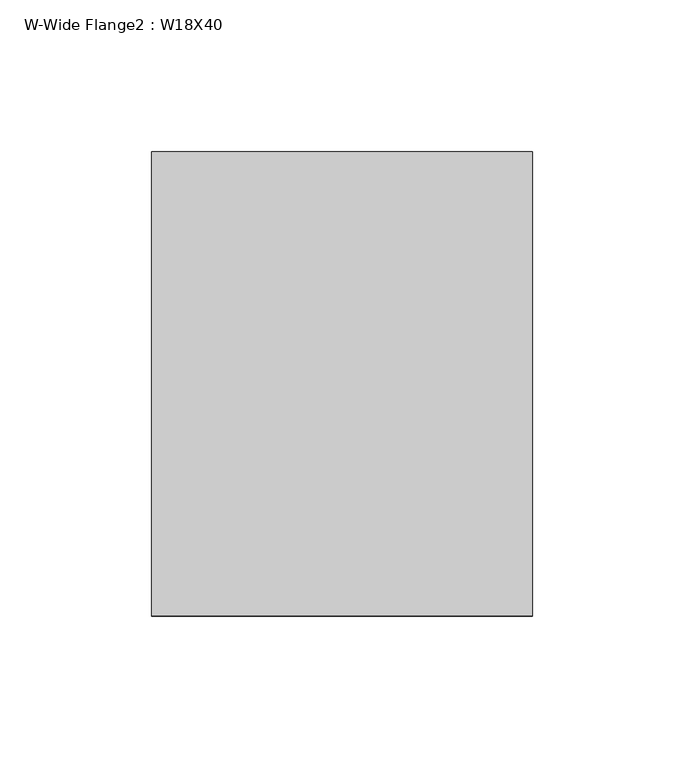
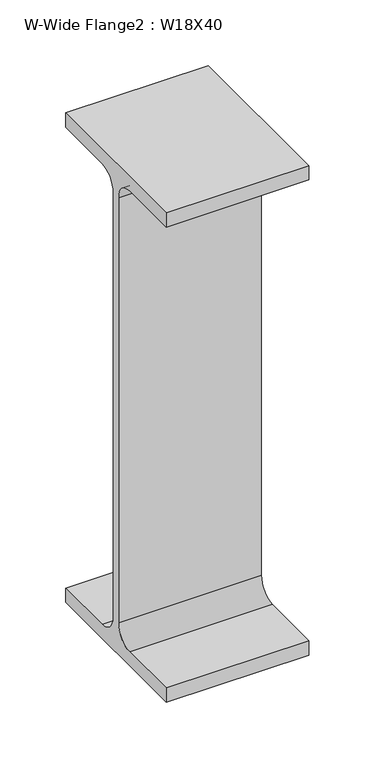
"""IFC4 building model written with IfcOpenShell, lengths in millimetres: beam geometry, W-Wide Flange2 : W18X40."""

from ifc_helpers import new_model, si_unit, point, frame, frame_2d, origin, place, context, project, spatial, polyline, circle_curve, trimmed, segment, composite_curve, outline, extrude, source, transform, mapped, element, save


def w_wide_flange2_w18x40_4b050a15(model_context):
    return source(origin(), model_context, "Body", "SweptSolid", [
        extrude(outline(composite_curve([segment(polyline([(76.454, -213.995), (76.454, -227.33), (-76.454, -227.33), (-76.454, -213.995), (-20.828, -213.995)]), True, "CONTINUOUS"), segment(trimmed(circle_curve(frame_2d((-20.828, -197.1675)), 16.8275), [point((-20.828, -213.995))], [point((-4.0005, -197.1675))], True, "CARTESIAN"), True, "CONTINUOUS"), segment(polyline([(-4.0005, -197.1675), (-4.0005, 197.1675)]), True, "CONTINUOUS"), segment(trimmed(circle_curve(frame_2d((-20.828, 197.1675)), 16.8275), [point((-4.0005, 197.1675))], [point((-20.828, 213.995))], True, "CARTESIAN"), True, "CONTINUOUS"), segment(polyline([(-20.828, 213.995), (-76.454, 213.995), (-76.454, 227.33), (76.454, 227.33), (76.454, 213.995), (20.828, 213.995)]), True, "CONTINUOUS"), segment(trimmed(circle_curve(frame_2d((20.828, 197.1675)), 16.8275), [point((20.828, 213.995))], [point((4.0005, 197.1675))], True, "CARTESIAN"), True, "CONTINUOUS"), segment(polyline([(4.0005, 197.1675), (4.0005, -197.1675)]), True, "CONTINUOUS"), segment(trimmed(circle_curve(frame_2d((20.828, -197.1675)), 16.8275), [point((4.0005, -197.1675))], [point((20.828, -213.995))], True, "CARTESIAN"), True, "CONTINUOUS"), segment(polyline([(20.828, -213.995), (76.454, -213.995)]), True, "CONTINUOUS")], self_intersect=False)), frame((-91.28125, 0.0, 0.0), z_axis=(1.0, 0.0, 0.0), x_axis=(0.0, 1.0, 0.0)), (0.0, 0.0, 1.0), 125.4125),
    ])


if __name__ == "__main__":
    model = new_model("IFC4")
    model_context = context("Model", 3, world=origin())
    ifc_project = project(units=[si_unit("LENGTHUNIT", "METRE", prefix="MILLI")], contexts=[model_context])
    site = spatial("IfcSite", under=ifc_project)
    building = spatial("IfcBuilding", under=site)
    placement = place(None, origin())
    w_wide_flange2_w18x40_shape = w_wide_flange2_w18x40_4b050a15(model_context)
    element("IfcBeam", 1, ObjectType="W-Wide Flange2 : W18X40", at=placement, inside=building, context=model_context, shape_type="MappedRepresentation", body=[
        mapped(w_wide_flange2_w18x40_shape, transform((0.0, 0.0, 0.0), x_axis=(1.0, 0.0, 0.0), y_axis=(0.0, 1.0, 0.0), z_axis=(0.0, 0.0, 1.0))),
    ])
    save(model, "model.ifc")

# Revit data of these elements
# Type "W-Wide Flange2 : W18X40"
#   Assembly Code = "B10"
#   W = 40
#   Length [instance default] = 5' - 0"
#   bf = 0' - 6.02"
#   d = 1' - 5.9"
#   k = 0' - 1 3/16"
#   k2 = 0' - 0.6625"
#   tf = 0' - 0.525"
#   tw = 0' - 0.315"
#   A = 0.0819444 SF
#   Structural Material [instance default] = Steel ASTM A992
# Element 1 (IfcBeam, "W-Wide Flange2 : W18X40")
#   Materials on its faces: "Steel ASTM A992"
# Materials
#   "Steel ASTM A992": class "Metal", colour RGB 199 199 199, transparency 0, Description = "Structural steel 50ksi", Cost = 0
